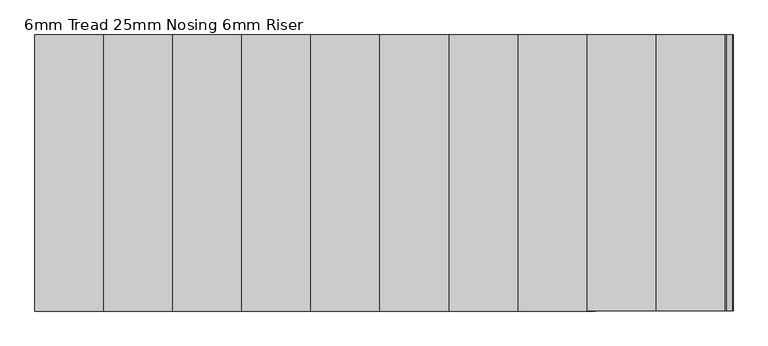
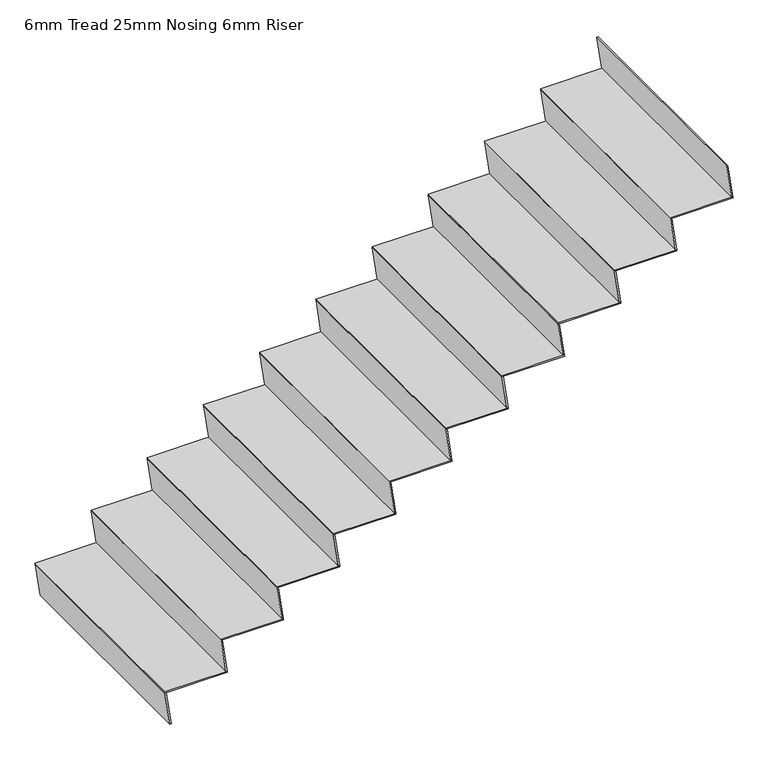
"""IFC4 building model written with IfcOpenShell, lengths in millimetres: stair flight geometry, 6mm Tread 25mm Nosing 6mm Riser."""

import ifcopenshell
import ifcopenshell.guid

model = None  # the IFC model being written
_history = None  # IfcOwnerHistory: only IFC2X3 demands one
_inside = {}  # id of a spatial element -> (the spatial element, [elements in it])
_under = {}  # id of a project, library or spatial element -> (it, [spatial elements below it])
_declared = {}  # id of a project -> (the project, [libraries it declares])
_typed = {}  # id of a type object -> (the type object, [elements of that type])
_made_of = {}  # id of a material, layer set ... -> (it, [elements and type objects made of it])


def new_model(schema):
    """Start an empty IFC model of exactly this schema.

    Asked for "IFC4X3", IfcOpenShell would pick the latest addendum, in which some entities
    have other attributes; the version numbers below select the first issue.
    IFC2X3 requires an IfcOwnerHistory on every rooted entity: one is made here for all.
    """
    global model, _history
    if schema == "IFC4X3":
        model = ifcopenshell.file(schema_version=(4, 3, 0, 0))
    else:
        model = ifcopenshell.file(schema=schema)
    _inside.clear()
    _under.clear()
    _declared.clear()
    _typed.clear()
    _made_of.clear()
    _history = None
    if model.schema == "IFC2X3":
        org = make("IfcOrganization", Name="unknown")
        user = make(
            "IfcPersonAndOrganization",
            ThePerson=make("IfcPerson", FamilyName="unknown"),
            TheOrganization=org,
        )
        app = make(
            "IfcApplication",
            ApplicationDeveloper=org,
            Version="unknown",
            ApplicationFullName="unknown",
            ApplicationIdentifier="unknown",
        )
        _history = make(
            "IfcOwnerHistory",
            OwningUser=user,
            OwningApplication=app,
            ChangeAction="ADDED",
            CreationDate=0,
        )
    return model


def make(cls, **values):
    """One entity of the class cls with the attributes given. An attribute that is None is left unset."""
    return model.create_entity(
        cls, **{name: value for name, value in values.items() if value is not None}
    )


def rooted(cls, **values):
    """An entity with a GlobalId (a new one), such as an element, a storey or a relation."""
    return make(cls, GlobalId=ifcopenshell.guid.new(), OwnerHistory=_history, **values)


def si_unit(unit_type, name, prefix=None):
    """IfcSIUnit, for example si_unit("LENGTHUNIT", "METRE", prefix="MILLI")."""
    return make("IfcSIUnit", UnitType=unit_type, Prefix=prefix, Name=name)


def assignment(units):
    """IfcUnitAssignment: the units of a project."""
    return None if units is None else make("IfcUnitAssignment", Units=units)


def point(xyz):
    """IfcCartesianPoint."""
    return None if xyz is None else make("IfcCartesianPoint", Coordinates=xyz)


def direction(xyz):
    """IfcDirection."""
    return None if xyz is None else make("IfcDirection", DirectionRatios=xyz)


def frame(location, z_axis=None, x_axis=None):
    """IfcAxis2Placement3D, a coordinate frame: its origin and axes. An axis left out is left unset."""
    return make(
        "IfcAxis2Placement3D",
        Location=point(location),
        Axis=direction(z_axis),
        RefDirection=direction(x_axis),
    )


def origin():
    """The frame at (0, 0, 0) with its axes left unset."""
    return frame((0.0, 0.0, 0.0))


def place(relative_to, where):
    """IfcLocalPlacement: puts the frame where relative to a parent placement (None: the world)."""
    return make(
        "IfcLocalPlacement", PlacementRelTo=relative_to, RelativePlacement=where
    )


def context(
    kind, dimensions, precision=None, world=None, true_north=None, identifier=None
):
    """IfcGeometricRepresentationContext, for example the 3D "Model" context."""
    return make(
        "IfcGeometricRepresentationContext",
        ContextIdentifier=identifier,
        ContextType=kind,
        CoordinateSpaceDimension=dimensions,
        Precision=precision,
        WorldCoordinateSystem=world,
        TrueNorth=true_north,
    )


def project(units=None, contexts=None):
    """IfcProject with its units and contexts."""
    return rooted(
        "IfcProject",
        Name="project",
        RepresentationContexts=contexts,
        UnitsInContext=assignment(units),
    )


def spatial(cls, under=None, at=None, **own):
    """A site, building, storey or space (cls), placed at a placement, below another one or the project."""
    s = rooted(cls, ObjectPlacement=at, **own)
    if under is not None:
        _under.setdefault(under.id(), (under, []))[1].append(s)
    return s


def polyline(points):
    """IfcPolyline through the points."""
    return make("IfcPolyline", Points=[point(p) for p in points])


def outline(outer, holes=None, kind="AREA"):
    """IfcArbitraryClosedProfileDef: a profile drawn as a closed curve; with holes, ...WithVoids."""
    if holes is None:
        return make("IfcArbitraryClosedProfileDef", ProfileType=kind, OuterCurve=outer)
    return make(
        "IfcArbitraryProfileDefWithVoids",
        ProfileType=kind,
        OuterCurve=outer,
        InnerCurves=holes,
    )


def extrude(swept, where, along, depth):
    """IfcExtrudedAreaSolid: the profile swept, set in the frame where, extruded along a direction by depth."""
    return make(
        "IfcExtrudedAreaSolid",
        SweptArea=swept,
        Position=where,
        ExtrudedDirection=direction(along),
        Depth=depth,
    )


def shape(context_of_items, identifier, shape_type, items):
    """IfcShapeRepresentation: the items that make up one representation, for example the "Body"."""
    return make(
        "IfcShapeRepresentation",
        ContextOfItems=context_of_items,
        RepresentationIdentifier=identifier,
        RepresentationType=shape_type,
        Items=items,
    )


def source(mapping_origin, context_of_items, identifier, shape_type, items):
    """IfcRepresentationMap: a shape defined once, which mapped items show again and again."""
    return make(
        "IfcRepresentationMap",
        MappingOrigin=mapping_origin,
        MappedRepresentation=shape(context_of_items, identifier, shape_type, items),
    )


def transform(
    local_origin,
    x_axis=None,
    y_axis=None,
    z_axis=None,
    scale=None,
    scale2=None,
    scale3=None,
    uniform=True,
):
    """IfcCartesianTransformationOperator3D, or its non-uniform kind. x_axis, y_axis, z_axis: its Axis1, 2, 3."""
    if uniform:
        return make(
            "IfcCartesianTransformationOperator3D",
            Axis1=direction(x_axis),
            Axis2=direction(y_axis),
            LocalOrigin=point(local_origin),
            Scale=scale,
            Axis3=direction(z_axis),
        )
    return make(
        "IfcCartesianTransformationOperator3DnonUniform",
        Axis1=direction(x_axis),
        Axis2=direction(y_axis),
        LocalOrigin=point(local_origin),
        Scale=scale,
        Axis3=direction(z_axis),
        Scale2=scale2,
        Scale3=scale3,
    )


def mapped(mapping_source, mapping_target):
    """IfcMappedItem: shows the shape of a source again, moved by a transform."""
    return make(
        "IfcMappedItem", MappingSource=mapping_source, MappingTarget=mapping_target
    )


def made_of(thing, what):
    """Note that an element or type object is made of a material, layer set ...; save() writes the relation."""
    if what is not None:
        _made_of.setdefault(what.id(), (what, []))[1].append(thing)
    return thing


def element(
    cls,
    number,
    at=None,
    inside=None,
    cuts=None,
    type_object=None,
    material=None,
    context=None,
    identifier="Body",
    shape_type=None,
    held_by="IfcProductDefinitionShape",
    body=None,
    shapes=None,
    **own,
):
    """One element of the class cls, such as IfcWall. Its Tag is "e" and its number.

    at: its placement. inside: the storey or other place that contains it. cuts: it is an
    opening in that element (IfcRelVoidsElement). A single representation is given by context,
    identifier, shape_type and body (its items); several are given by shapes. held_by: the class
    of the entity that holds the representations. save() writes the other relations.
    """
    e = rooted(cls, Tag="e%d" % number, ObjectPlacement=at, **own)
    if body is not None:
        shapes = [shape(context, identifier, shape_type, body)]
    if shapes is not None:
        e.Representation = make(held_by, Representations=shapes)
    if inside is not None:
        _inside.setdefault(inside.id(), (inside, []))[1].append(e)
    if cuts is not None:
        rooted(
            "IfcRelVoidsElement", RelatingBuildingElement=cuts, RelatedOpeningElement=e
        )
    if type_object is not None:
        _typed.setdefault(type_object.id(), (type_object, []))[1].append(e)
    return made_of(e, material)


def aggregate(whole, parts):
    """IfcRelAggregates: a whole, such as a stair, and the parts it consists of."""
    return rooted("IfcRelAggregates", RelatingObject=whole, RelatedObjects=parts)


def save(model, path):
    """Write the relations noted so far, then the file.

    IfcRelAggregates (storeys below a building ...), IfcRelContainedInSpatialStructure (elements
    in a storey), IfcRelDefinesByType, IfcRelAssociatesMaterial and IfcRelDeclares: one each for
    every whole, place, type object, material and project.
    """
    for whole, parts in _under.values():
        aggregate(whole, parts)
    for where, things in _inside.values():
        rooted(
            "IfcRelContainedInSpatialStructure",
            RelatedElements=things,
            RelatingStructure=where,
        )
    for kind, things in _typed.values():
        rooted("IfcRelDefinesByType", RelatedObjects=things, RelatingType=kind)
    for what, things in _made_of.values():
        rooted("IfcRelAssociatesMaterial", RelatedObjects=things, RelatingMaterial=what)
    for by, libraries in _declared.values():
        rooted("IfcRelDeclares", RelatingContext=by, RelatedDefinitions=libraries)
    model.write(path)


def stair_flight_6mm_tread_25mm_nosing_6mm_riser_9854de60(model_context):
    return source(origin(), model_context, "Body", "SweptSolid", [
        extrude(outline(polyline([(8176.4705882, 13906.0599092), (8176.4705882, 13600.0), (8170.4705882, 13600.85), (8170.4705882, 13906.9099092), (8176.4705882, 13906.0599092)])), frame((0.0, 10370.4345331, 0.0), z_axis=(0.0, 1.0, 0.0), x_axis=(0.0, 0.0, 1.0)), (0.0, 0.0, 1.0), 1100.0),
        extrude(outline(polyline([(8170.4705882, 13600.85), (8000.0, 13625.0), (8000.0, 13631.0599092), (8170.4705882, 13606.9099092), (8170.4705882, 13600.85)])), frame((0.0, 10370.4345331, 0.0), z_axis=(0.0, 1.0, 0.0), x_axis=(0.0, 0.0, 1.0)), (0.0, 0.0, 1.0), 1100.0),
        extrude(outline(polyline([(8346.9411765, 13875.85), (8176.4705882, 13900.0), (8176.4705882, 13906.0599092), (8346.9411765, 13881.9099092), (8346.9411765, 13875.85)])), frame((0.0, 10370.4345331, 0.0), z_axis=(0.0, 1.0, 0.0), x_axis=(0.0, 0.0, 1.0)), (0.0, 0.0, 1.0), 1100.0),
        extrude(outline(polyline([(8352.9411765, 14181.0599092), (8352.9411765, 13875.0), (8346.9411765, 13875.85), (8346.9411765, 14181.9099092), (8352.9411765, 14181.0599092)])), frame((0.0, 10370.4345331, 0.0), z_axis=(0.0, 1.0, 0.0), x_axis=(0.0, 0.0, 1.0)), (0.0, 0.0, 1.0), 1100.0),
        extrude(outline(polyline([(8523.4117647, 14150.85), (8352.9411765, 14175.0), (8352.9411765, 14181.0599092), (8523.4117647, 14156.9099092), (8523.4117647, 14150.85)])), frame((0.0, 10370.4345331, 0.0), z_axis=(0.0, 1.0, 0.0), x_axis=(0.0, 0.0, 1.0)), (0.0, 0.0, 1.0), 1100.0),
        extrude(outline(polyline([(8529.4117647, 14456.0599092), (8529.4117647, 14150.0), (8523.4117647, 14150.85), (8523.4117647, 14456.9099092), (8529.4117647, 14456.0599092)])), frame((0.0, 10370.4345331, 0.0), z_axis=(0.0, 1.0, 0.0), x_axis=(0.0, 0.0, 1.0)), (0.0, 0.0, 1.0), 1100.0),
        extrude(outline(polyline([(8699.8823529, 14425.85), (8529.4117647, 14450.0), (8529.4117647, 14456.0599092), (8699.8823529, 14431.9099092), (8699.8823529, 14425.85)])), frame((0.0, 10370.4345331, 0.0), z_axis=(0.0, 1.0, 0.0), x_axis=(0.0, 0.0, 1.0)), (0.0, 0.0, 1.0), 1100.0),
        extrude(outline(polyline([(8705.8823529, 14731.0599092), (8705.8823529, 14425.0), (8699.8823529, 14425.85), (8699.8823529, 14731.9099092), (8705.8823529, 14731.0599092)])), frame((0.0, 10370.4345331, 0.0), z_axis=(0.0, 1.0, 0.0), x_axis=(0.0, 0.0, 1.0)), (0.0, 0.0, 1.0), 1100.0),
        extrude(outline(polyline([(8876.3529412, 14700.85), (8705.8823529, 14725.0), (8705.8823529, 14731.0599092), (8876.3529412, 14706.9099092), (8876.3529412, 14700.85)])), frame((0.0, 10370.4345331, 0.0), z_axis=(0.0, 1.0, 0.0), x_axis=(0.0, 0.0, 1.0)), (0.0, 0.0, 1.0), 1100.0),
        extrude(outline(polyline([(8882.3529412, 15006.0599092), (8882.3529412, 14700.0), (8876.3529412, 14700.85), (8876.3529412, 15006.9099092), (8882.3529412, 15006.0599092)])), frame((0.0, 10370.4345331, 0.0), z_axis=(0.0, 1.0, 0.0), x_axis=(0.0, 0.0, 1.0)), (0.0, 0.0, 1.0), 1100.0),
        extrude(outline(polyline([(9052.8235294, 14975.85), (8882.3529412, 15000.0), (8882.3529412, 15006.0599092), (9052.8235294, 14981.9099092), (9052.8235294, 14975.85)])), frame((0.0, 10370.4345331, 0.0), z_axis=(0.0, 1.0, 0.0), x_axis=(0.0, 0.0, 1.0)), (0.0, 0.0, 1.0), 1100.0),
        extrude(outline(polyline([(9058.8235294, 15281.0599092), (9058.8235294, 14975.0), (9052.8235294, 14975.85), (9052.8235294, 15281.9099092), (9058.8235294, 15281.0599092)])), frame((0.0, 10370.4345331, 0.0), z_axis=(0.0, 1.0, 0.0), x_axis=(0.0, 0.0, 1.0)), (0.0, 0.0, 1.0), 1100.0),
        extrude(outline(polyline([(9229.2941176, 15250.85), (9058.8235294, 15275.0), (9058.8235294, 15281.0599092), (9229.2941176, 15256.9099092), (9229.2941176, 15250.85)])), frame((0.0, 10370.4345331, 0.0), z_axis=(0.0, 1.0, 0.0), x_axis=(0.0, 0.0, 1.0)), (0.0, 0.0, 1.0), 1100.0),
        extrude(outline(polyline([(9235.2941176, 15556.0599092), (9235.2941176, 15250.0), (9229.2941176, 15250.85), (9229.2941176, 15556.9099092), (9235.2941176, 15556.0599092)])), frame((0.0, 10370.4345331, 0.0), z_axis=(0.0, 1.0, 0.0), x_axis=(0.0, 0.0, 1.0)), (0.0, 0.0, 1.0), 1100.0),
        extrude(outline(polyline([(9405.7647059, 15525.85), (9235.2941176, 15550.0), (9235.2941176, 15556.0599092), (9405.7647059, 15531.9099092), (9405.7647059, 15525.85)])), frame((0.0, 10370.4345331, 0.0), z_axis=(0.0, 1.0, 0.0), x_axis=(0.0, 0.0, 1.0)), (0.0, 0.0, 1.0), 1100.0),
        extrude(outline(polyline([(9411.7647059, 15831.0599092), (9411.7647059, 15525.0), (9405.7647059, 15525.85), (9405.7647059, 15831.9099092), (9411.7647059, 15831.0599092)])), frame((0.0, 10370.4345331, 0.0), z_axis=(0.0, 1.0, 0.0), x_axis=(0.0, 0.0, 1.0)), (0.0, 0.0, 1.0), 1100.0),
        extrude(outline(polyline([(9582.2352941, 15800.85), (9411.7647059, 15825.0), (9411.7647059, 15831.0599092), (9582.2352941, 15806.9099092), (9582.2352941, 15800.85)])), frame((0.0, 10370.4345331, 0.0), z_axis=(0.0, 1.0, 0.0), x_axis=(0.0, 0.0, 1.0)), (0.0, 0.0, 1.0), 1100.0),
        extrude(outline(polyline([(9588.2352941, 16106.0599092), (9588.2352941, 15800.0), (9582.2352941, 15800.85), (9582.2352941, 16106.9099092), (9588.2352941, 16106.0599092)])), frame((0.0, 10370.4345331, 0.0), z_axis=(0.0, 1.0, 0.0), x_axis=(0.0, 0.0, 1.0)), (0.0, 0.0, 1.0), 1100.0),
        extrude(outline(polyline([(9758.7058824, 16075.85), (9588.2352941, 16100.0), (9588.2352941, 16106.0599092), (9758.7058824, 16081.9099092), (9758.7058824, 16075.85)])), frame((0.0, 10370.4345331, 0.0), z_axis=(0.0, 1.0, 0.0), x_axis=(0.0, 0.0, 1.0)), (0.0, 0.0, 1.0), 1100.0),
        extrude(outline(polyline([(9764.7058824, 16381.0599092), (9764.7058824, 16075.0), (9758.7058824, 16075.85), (9758.7058824, 16381.9099092), (9764.7058824, 16381.0599092)])), frame((0.0, 10370.4345331, 0.0), z_axis=(0.0, 1.0, 0.0), x_axis=(0.0, 0.0, 1.0)), (0.0, 0.0, 1.0), 1100.0),
        extrude(outline(polyline([(9935.1764706, 16350.85), (9764.7058824, 16375.0), (9764.7058824, 16381.0599092), (9935.1764706, 16356.9099092), (9935.1764706, 16350.85)])), frame((0.0, 10370.4345331, 0.0), z_axis=(0.0, 1.0, 0.0), x_axis=(0.0, 0.0, 1.0)), (0.0, 0.0, 1.0), 1100.0),
    ])


if __name__ == "__main__":
    model = new_model("IFC4")
    model_context = context("Model", 3, world=origin())
    ifc_project = project(units=[si_unit("LENGTHUNIT", "METRE", prefix="MILLI")], contexts=[model_context])
    site = spatial("IfcSite", under=ifc_project)
    building = spatial("IfcBuilding", under=site)
    placement = place(None, origin())
    stair_flight_6mm_tread_25mm_nosing_6mm_riser_shape = stair_flight_6mm_tread_25mm_nosing_6mm_riser_9854de60(model_context)
    element("IfcStairFlight", 1, ObjectType="6mm Tread 25mm Nosing 6mm Riser", at=placement, inside=building, context=model_context, shape_type="MappedRepresentation", body=[
        mapped(stair_flight_6mm_tread_25mm_nosing_6mm_riser_shape, transform((0.0, 0.0, 0.0), x_axis=(1.0, 0.0, 0.0), y_axis=(0.0, 1.0, 0.0), z_axis=(0.0, 0.0, 1.0))),
    ])
    save(model, "model.ifc")

# Revit data of these elements
# Element 1 (IfcStairFlight, "6mm Tread 25mm Nosing 6mm Riser")
#   Materials on its faces: "Steel, Paint Finish, Dark Gray"
# Materials
#   "Steel, Paint Finish, Dark Gray": class "Metal", colour RGB 89 89 89, transparency 0, Description = "Steel, paint finish, dark gray, glossy", Cost = 0
